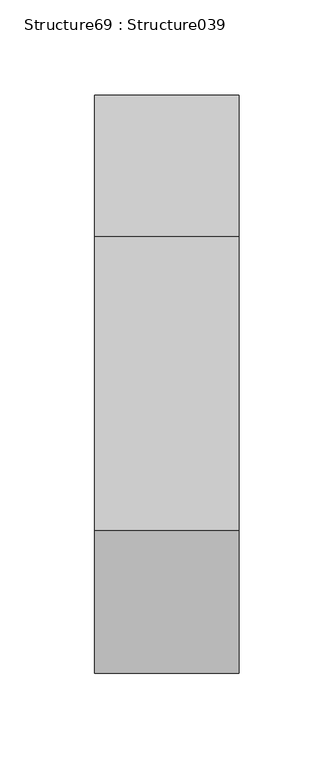
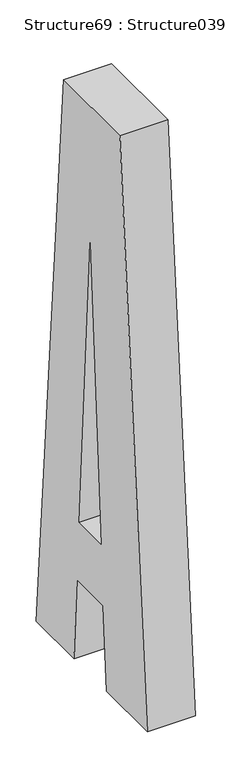
"""IFC4 building model written with IfcOpenShell, lengths in millimetres: proxy geometry, Structure69 : Structure039."""

from ifc_helpers import new_model, si_unit, frame, origin, place, context, project, spatial, polyline, outline, extrude, source, transform, mapped, element, save


def structure69_structure039_35aea155(model_context):
    return source(origin(), model_context, "Body", "SweptSolid", [
        extrude(outline(polyline([(283977.4343092, 3528.5825142), (283874.0833829, 3528.5825142), (283865.9383689, 3665.9109904), (283793.8632133, 3665.9109904), (283784.3345608, 3528.5825142), (283672.8442885, 3528.5825142), (283747.6243722, 4480.4419946), (283902.6447787, 4480.4419946), (283977.4343092, 3528.5825142)]), holes=[polyline([(283860.4913553, 3765.1859458), (283830.5702529, 4250.6490619), (283799.3032992, 3765.1859458), (283860.4913553, 3765.1859458)])]), frame((-59031.6926606, 0.0, 0.0), z_axis=(1.0, 0.0, 0.0), x_axis=(0.0, 1.0, 0.0)), (0.0, 0.0, 1.0), 76.2),
    ])


if __name__ == "__main__":
    model = new_model("IFC4")
    model_context = context("Model", 3, world=origin())
    ifc_project = project(units=[si_unit("LENGTHUNIT", "METRE", prefix="MILLI")], contexts=[model_context])
    site = spatial("IfcSite", under=ifc_project)
    building = spatial("IfcBuilding", under=site)
    placement = place(None, origin())
    structure69_structure039_shape = structure69_structure039_35aea155(model_context)
    element("IfcBuildingElementProxy", 1, Name="Structure69 : Structure039", ObjectType="Structure69 : Structure039", at=placement, inside=building, context=model_context, shape_type="MappedRepresentation", body=[
        mapped(structure69_structure039_shape, transform((0.0, 0.0, 0.0), x_axis=(1.0, 0.0, 0.0), y_axis=(0.0, 1.0, 0.0), z_axis=(0.0, 0.0, 1.0))),
    ])
    save(model, "model.ifc")

# Revit data of these elements
# Type "Structure69 : Structure039"
#   NameOverride = "Structure039"
# Element 1 (IfcBuildingElementProxy, "Structure69 : Structure039")
#   Materials on its faces: "BRUSHED ALUM. LETTERING"
# Materials
#   "BRUSHED ALUM. LETTERING": class "Unassigned", colour RGB 169 181 186, transparency 0, Cost = 0
